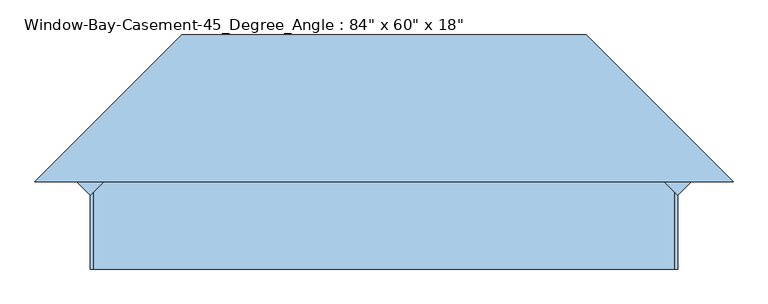
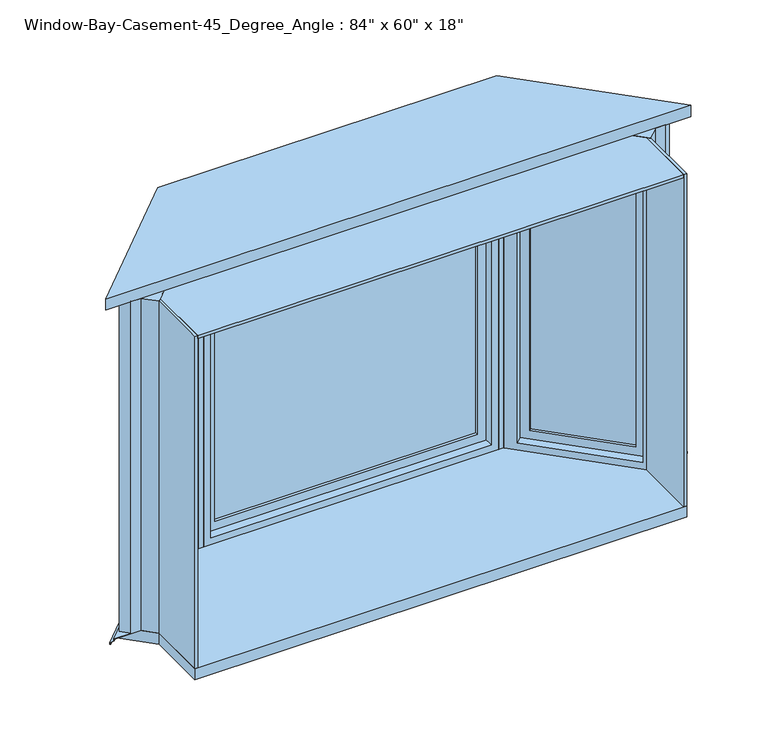
"""IFC4 building model written with IfcOpenShell, lengths in millimetres: window geometry."""

from ifc_helpers import new_model, si_unit, frame, origin, place, context, project, spatial, polyline, outline, extrude, faceted_brep, source, transform, mapped, element, save


def window_a80803ce(model_context):
    return source(origin(), model_context, "Body", "SolidModel", [
        extrude(outline(polyline([(1066.8, 208.1414087), (1062.3098719, 203.6512806), (771.5637138, 494.3974388), (776.0538418, 498.8875668), (1066.8, 208.1414087)])), frame((0.0, 0.0, 730.25), z_axis=(0.0, 0.0, 1.0), x_axis=(1.0, 0.0, 0.0)), (0.0, 0.0, 1.0), 1384.3),
        extrude(outline(polyline([(1057.8197439, 199.1611525), (1053.3296158, 194.6710245), (762.5834576, 485.4171827), (767.0735857, 489.9073107), (1057.8197439, 199.1611525)])), frame((0.0, 0.0, 730.25), z_axis=(0.0, 0.0, 1.0), x_axis=(1.0, 0.0, 0.0)), (0.0, 0.0, 1.0), 1384.3),
        extrude(outline(polyline([(1441.45, 57.15), (1441.45, -468.3271601), (-57.15, -468.3271601), (-57.15, 57.15), (1441.45, 57.15)]), holes=[polyline([(1384.3, -411.1771601), (1384.3, 0.0), (0.0, 0.0), (0.0, -411.1771601), (1384.3, -411.1771601)])]), frame((1044.3493597, 185.6907684, 730.25), z_axis=(0.7071067811865468, 0.7071067811865483, 0.0), x_axis=(0.0, 0.0, 1.0)), (0.0, 0.0, 1.0), 44.45),
        faceted_brep([(661.8085913, 514.35, 2184.4), (1066.8, 109.3585913, 2184.4), (1116.1914087, 158.75, 2184.4), (1161.0926893, 158.75, 2184.4), (703.8926893, 615.95, 2184.4), (1084.7605122, 145.2796158, 2171.7), (713.192049, 516.8480791, 2171.7), (758.0933296, 561.7493597, 2171.7), (1129.6617928, 190.1808964, 2171.7), (1044.3493597, 131.8092316, 2152.65), (699.7216648, 476.4369265, 2152.65), (726.6624332, 503.3776949, 2152.65), (1071.2901281, 158.75, 2152.65), (713.192049, 516.8480791, 673.1), (758.0933296, 561.7493597, 673.1), (699.7216648, 476.4369265, 692.15), (726.6624332, 503.3776949, 692.15), (703.8926893, 615.95, 660.4), (1161.0926893, 158.75, 660.4), (1116.1914087, 158.75, 660.4), (1066.8, 109.3585913, 660.4), (661.8085913, 514.35, 660.4), (1084.7605122, 145.2796158, 673.1), (1129.6617928, 190.1808964, 673.1), (1044.3493597, 131.8092316, 692.15), (1071.2901281, 158.75, 692.15)], [[[0, 1, 2, 3, 4]], [[5, 6, 7, 8]], [[9, 10, 11, 12]], [[6, 13, 14, 7]], [[10, 15, 16, 11]], [[17, 18, 19, 20, 21]], [[13, 22, 23, 14]], [[15, 24, 25, 16]], [[20, 19, 2, 1]], [[3, 18, 17, 4], [7, 14, 23, 8]], [[8, 23, 22, 5]], [[5, 22, 13, 6], [11, 16, 25, 12]], [[12, 25, 24, 9]], [[1, 0, 21, 20], [9, 24, 15, 10]], [[4, 17, 21, 0]], [[2, 19, 18, 3]]]),
        extrude(outline(polyline([(-1066.8, 208.1414087), (-776.0538418, 498.8875668), (-771.5637138, 494.3974388), (-1062.3098719, 203.6512806), (-1066.8, 208.1414087)])), frame((0.0, 0.0, 730.25), z_axis=(0.0, 0.0, 1.0), x_axis=(1.0, 0.0, 0.0)), (0.0, 0.0, 1.0), 1384.3),
        extrude(outline(polyline([(-1057.8197439, 199.1611525), (-767.0735857, 489.9073107), (-762.5834576, 485.4171827), (-1053.3296158, 194.6710245), (-1057.8197439, 199.1611525)])), frame((0.0, 0.0, 730.25), z_axis=(0.0, 0.0, 1.0), x_axis=(1.0, 0.0, 0.0)), (0.0, 0.0, 1.0), 1384.3),
        extrude(outline(polyline([(1441.45, -57.15), (-57.15, -57.15), (-57.15, 468.3271601), (1441.45, 468.3271601), (1441.45, -57.15)]), holes=[polyline([(1384.3, 411.1771601), (0.0, 411.1771601), (0.0, 0.0), (1384.3, 0.0), (1384.3, 411.1771601)])]), frame((-1044.3493597, 185.6907684, 730.25), z_axis=(-0.7071067811865468, 0.7071067811865483, 0.0), x_axis=(0.0, 0.0, 1.0)), (0.0, 0.0, 1.0), 44.45),
        faceted_brep([(-661.8085913, 514.35, 2184.4), (-703.8926893, 615.95, 2184.4), (-1161.0926893, 158.75, 2184.4), (-1116.1914087, 158.75, 2184.4), (-1066.8, 109.3585913, 2184.4), (-1084.7605122, 145.2796158, 2171.7), (-1129.6617928, 190.1808964, 2171.7), (-758.0933296, 561.7493597, 2171.7), (-713.192049, 516.8480791, 2171.7), (-1044.3493597, 131.8092316, 2152.65), (-1071.2901281, 158.75, 2152.65), (-726.6624332, 503.3776949, 2152.65), (-699.7216648, 476.4369265, 2152.65), (-758.0933296, 561.7493597, 673.1), (-713.192049, 516.8480791, 673.1), (-726.6624332, 503.3776949, 692.15), (-699.7216648, 476.4369265, 692.15), (-703.8926893, 615.95, 660.4), (-661.8085913, 514.35, 660.4), (-1066.8, 109.3585913, 660.4), (-1116.1914087, 158.75, 660.4), (-1161.0926893, 158.75, 660.4), (-1129.6617928, 190.1808964, 673.1), (-1084.7605122, 145.2796158, 673.1), (-1071.2901281, 158.75, 692.15), (-1044.3493597, 131.8092316, 692.15)], [[[0, 1, 2, 3, 4]], [[5, 6, 7, 8]], [[9, 10, 11, 12]], [[8, 7, 13, 14]], [[12, 11, 15, 16]], [[17, 18, 19, 20, 21]], [[14, 13, 22, 23]], [[16, 15, 24, 25]], [[19, 4, 3, 20]], [[2, 1, 17, 21], [7, 6, 22, 13]], [[6, 5, 23, 22]], [[5, 8, 14, 23], [11, 10, 24, 15]], [[10, 9, 25, 24]], [[4, 19, 18, 0], [9, 12, 16, 25]], [[1, 0, 18, 17]], [[3, 2, 21, 20]]]),
        faceted_brep([(-724.9347382, 666.75, 660.4), (-724.9347382, 666.75, 653.0697935), (724.9347382, 666.75, 653.0697935), (724.9347382, 666.75, 660.4), (-703.8926893, 615.95, 663.1486341), (-703.8926893, 615.95, 660.4), (703.8926893, 615.95, 660.4), (703.8926893, 615.95, 663.1486341), (-725.5133946, 668.147, 654.4483503), (-725.5133946, 668.147, 663.1486341), (725.5133946, 668.147, 663.1486341), (725.5133946, 668.147, 654.4483503), (730.7739068, 680.847, 652.2089977), (-730.7739068, 680.847, 652.2089977), (730.7739068, 680.847, 643.2668038), (-730.7739068, 680.847, 643.2668038), (-729.132627, 676.8846, 644.7270038), (-729.132627, 676.8846, 643.2668038), (729.132627, 676.8846, 643.2668038), (729.132627, 676.8846, 644.7270038), (-730.1110823, 679.2468, 650.8662705), (-730.1110823, 679.2468, 644.7270038), (730.1110823, 679.2468, 644.7270038), (730.1110823, 679.2468, 650.8662705), (-1232.9347382, 158.75, 660.4), (-1232.9347382, 158.75, 653.0697935), (1232.9347382, 158.75, 660.4), (1161.0926893, 158.75, 660.4), (-1161.0926893, 158.75, 660.4), (-1161.0926893, 158.75, 663.1486341), (1161.0926893, 158.75, 663.1486341), (1234.9103945, 158.75, 663.1486341), (-1234.9103945, 158.75, 663.1486341), (-1234.9103945, 158.75, 654.4483503), (-1252.8709068, 158.75, 652.2089977), (-1252.8709068, 158.75, 643.2668038), (1252.8709068, 158.75, 643.2668038), (1247.2672271, 158.75, 643.2668038), (-1247.2672271, 158.75, 643.2668038), (-1247.2672271, 158.75, 644.7270038), (1247.2672271, 158.75, 644.7270038), (1250.6078823, 158.75, 644.7270038), (-1250.6078823, 158.75, 644.7270038), (-1250.6078823, 158.75, 650.8662705), (1232.9347382, 158.75, 653.0697935), (1234.9103945, 158.75, 654.4483503), (1252.8709068, 158.75, 652.2089977), (1250.6078823, 158.75, 650.8662705)], [[[0, 1, 2, 3]], [[4, 5, 6, 7]], [[8, 9, 10, 11]], [[8, 11, 12, 13]], [[13, 12, 14, 15]], [[16, 17, 18, 19]], [[20, 21, 22, 23]], [[2, 1, 20, 23]], [[1, 0, 24, 25]], [[0, 3, 26, 27, 6, 5, 28, 24]], [[5, 4, 29, 28]], [[4, 7, 30, 31, 10, 9, 32, 29]], [[9, 8, 33, 32]], [[8, 13, 34, 33]], [[13, 15, 35, 34]], [[15, 14, 36, 37, 18, 17, 38, 35]], [[17, 16, 39, 38]], [[16, 19, 40, 41, 22, 21, 42, 39]], [[21, 20, 43, 42]], [[20, 1, 25, 43]], [[3, 2, 44, 26]], [[7, 6, 27, 30]], [[11, 10, 31, 45]], [[12, 11, 45, 46]], [[14, 12, 46, 36]], [[19, 18, 37, 40]], [[23, 22, 41, 47]], [[2, 23, 47, 44]], [[25, 24, 28, 29, 32, 33, 34, 35, 38, 39, 42, 43]], [[27, 26, 44, 47, 41, 40, 37, 36, 46, 45, 31, 30]]]),
        extrude(outline(polyline([(-1138.642049, 181.2006403), (-1161.0926893, 158.75), (-1192.5235857, 190.1808964), (-1170.0729454, 212.6315367), (-1138.642049, 181.2006403)])), frame((0.0, 0.0, 663.1486341), z_axis=(0.0, 0.0, 1.0), x_axis=(1.0, 0.0, 0.0)), (0.0, 0.0, 1.0), 1521.2513659),
        extrude(outline(polyline([(1138.642049, 181.2006403), (1170.0729454, 212.6315367), (1192.5235857, 190.1808964), (1161.0926893, 158.75), (1138.642049, 181.2006403)])), frame((0.0, 0.0, 663.1486341), z_axis=(0.0, 0.0, 1.0), x_axis=(1.0, 0.0, 0.0)), (0.0, 0.0, 1.0), 1521.2513659),
        extrude(outline(polyline([(-661.8085913, 514.35), (661.8085913, 514.35), (1054.1, 122.0585913), (1054.1, -158.75), (-1054.1, -158.75), (-1054.1, 122.0585913), (-661.8085913, 514.35)])), frame((0.0, 0.0, 2171.7), z_axis=(0.0, 0.0, 1.0), x_axis=(1.0, 0.0, 0.0)), (0.0, 0.0, 1.0), 12.7),
        extrude(outline(polyline([(-1066.8, -158.75), (-1066.8, 109.3585913), (-1054.1, 122.0585913), (-1054.1, -158.75), (-1066.8, -158.75)])), frame((0.0, 0.0, 660.4), z_axis=(0.0, 0.0, 1.0), x_axis=(1.0, 0.0, 0.0)), (0.0, 0.0, 1.0), 1524.0),
        extrude(outline(polyline([(1066.8, -158.75), (1054.1, -158.75), (1054.1, 122.0585913), (1066.8, 109.3585913), (1066.8, -158.75)])), frame((0.0, 0.0, 660.4), z_axis=(0.0, 0.0, 1.0), x_axis=(1.0, 0.0, 0.0)), (0.0, 0.0, 1.0), 1524.0),
        extrude(outline(polyline([(2171.7, -627.2414087), (673.1, -627.2414087), (673.1, 627.2414087), (2171.7, 627.2414087), (2171.7, -627.2414087)]), holes=[polyline([(2114.55, 570.0914087), (730.25, 570.0914087), (730.25, -570.0914087), (2114.55, -570.0914087), (2114.55, 570.0914087)])]), frame((0.0, 552.45, 0.0), z_axis=(0.0, 1.0, 0.0), x_axis=(0.0, 0.0, 1.0)), (0.0, 0.0, 1.0), 44.45),
        extrude(outline(polyline([(1066.8, -158.75), (-1066.8, -158.75), (-1066.8, 109.3585913), (-1174.5630735, 217.1216648), (-724.9347382, 666.75), (724.9347382, 666.75), (1174.5630735, 217.1216648), (1066.8, 109.3585913), (1066.8, -158.75)])), frame((0.0, 0.0, 609.6), z_axis=(0.0, 0.0, 1.0), x_axis=(1.0, 0.0, 0.0)), (0.0, 0.0, 1.0), 50.8),
        extrude(outline(polyline([(570.0914087, 584.2), (570.0914087, 577.85), (-570.0914087, 577.85), (-570.0914087, 584.2), (570.0914087, 584.2)])), frame((0.0, 0.0, 730.25), z_axis=(0.0, 0.0, 1.0), x_axis=(1.0, 0.0, 0.0)), (0.0, 0.0, 1.0), 1384.3),
        extrude(outline(polyline([(570.0914087, 571.5), (570.0914087, 565.15), (-570.0914087, 565.15), (-570.0914087, 571.5), (570.0914087, 571.5)])), frame((0.0, 0.0, 730.25), z_axis=(0.0, 0.0, 1.0), x_axis=(1.0, 0.0, 0.0)), (0.0, 0.0, 1.0), 1384.3),
        faceted_brep([(627.2414087, 552.45, 673.1), (627.2414087, 615.95, 673.1), (-627.2414087, 615.95, 673.1), (-627.2414087, 552.45, 673.1), (608.1914087, 514.35, 692.15), (608.1914087, 552.45, 692.15), (-608.1914087, 552.45, 692.15), (-608.1914087, 514.35, 692.15), (639.9414087, 615.95, 660.4), (639.9414087, 514.35, 660.4), (-639.9414087, 514.35, 660.4), (-639.9414087, 615.95, 660.4), (-627.2414087, 615.95, 2171.7), (-627.2414087, 552.45, 2171.7), (-608.1914087, 552.45, 2152.65), (-608.1914087, 514.35, 2152.65), (-639.9414087, 514.35, 2184.4), (-639.9414087, 615.95, 2184.4), (627.2414087, 615.95, 2171.7), (627.2414087, 552.45, 2171.7), (608.1914087, 552.45, 2152.65), (608.1914087, 514.35, 2152.65), (639.9414087, 514.35, 2184.4), (639.9414087, 615.95, 2184.4)], [[[0, 1, 2, 3]], [[4, 5, 6, 7]], [[8, 9, 10, 11]], [[3, 2, 12, 13]], [[7, 6, 14, 15]], [[11, 10, 16, 17]], [[13, 12, 18, 19]], [[15, 14, 20, 21]], [[17, 16, 22, 23]], [[11, 17, 23, 8], [1, 18, 12, 2]], [[19, 18, 1, 0]], [[3, 13, 19, 0], [5, 20, 14, 6]], [[21, 20, 5, 4]], [[9, 22, 16, 10], [7, 15, 21, 4]], [[23, 22, 9, 8]]]),
        extrude(outline(polyline([(-639.9414087, 615.95), (-639.9414087, 514.35), (-661.8085913, 514.35), (-703.8926893, 615.95), (-639.9414087, 615.95)])), frame((0.0, 0.0, 660.4), z_axis=(0.0, 0.0, 1.0), x_axis=(1.0, 0.0, 0.0)), (0.0, 0.0, 1.0), 1524.0),
        extrude(outline(polyline([(703.8926893, 615.95), (661.8085913, 514.35), (639.9414087, 514.35), (639.9414087, 615.95), (703.8926893, 615.95)])), frame((0.0, 0.0, 660.4), z_axis=(0.0, 0.0, 1.0), x_axis=(1.0, 0.0, 0.0)), (0.0, 0.0, 1.0), 1524.0),
        extrude(outline(polyline([(735.4557627, 692.15), (1268.8557627, 158.75), (-1268.8557627, 158.75), (-735.4557627, 692.15), (735.4557627, 692.15)])), frame((0.0, 0.0, 2184.4), z_axis=(0.0, 0.0, 1.0), x_axis=(1.0, 0.0, 0.0)), (0.0, 0.0, 1.0), 50.8),
    ])


if __name__ == "__main__":
    model = new_model("IFC4")
    model_context = context("Model", 3, world=origin())
    ifc_project = project(units=[si_unit("LENGTHUNIT", "METRE", prefix="MILLI")], contexts=[model_context])
    site = spatial("IfcSite", under=ifc_project)
    building = spatial("IfcBuilding", under=site)
    placement = place(None, origin())
    window_shape = window_a80803ce(model_context)
    element("IfcWindow", 1, ObjectType="Window-Bay-Casement-45_Degree_Angle : 84\" x 60\" x 18\"", at=placement, inside=building, context=model_context, shape_type="MappedRepresentation", body=[
        mapped(window_shape, transform((0.0, 0.0, 0.0), x_axis=(1.0, 0.0, 0.0), y_axis=(0.0, 1.0, 0.0), z_axis=(0.0, 0.0, 1.0))),
    ])
    save(model, "model.ifc")

# Revit data of these elements
# Type "Window-Bay-Casement-45_Degree_Angle : 84\" x 60\" x 18\""
#   Type Mark = "27"
#   Fire Rating = "0.5h"
#   Assembly Code = "B2020100"
#   Analytic Construction = "Double glazing - domestic"
#   Width of Middle Sash = 4' - 2.38909"
#   Width = 7' - 0"
#   Visual Light Transmittance = 0.81
#   Thermal Resistance (R) = 1.8146 (h·ft²·°F)/BTU
#   Solar Heat Gain Coefficient = 0.76
#   Rough Width = 7' - 0 1/2"
#   Rough Height = 5' - 0 1/2"
#   Length 4 = 0' - 1.13909"
#   Length 3 = 0' - 0.51777"
#   Length 2 = 4' - 7.42462"
#   Length 1 = 1' - 2.80546"
#   Wall Thickness [instance default] = 0' - 6"
#   Trim Width = 7' - 5.03553"
#   Trim Height = 5' - 0"
#   Height 1 = 5' - 2"
#   Height = 5' - 0"
#   Heat Transfer Coefficient (U) = 0.5511 BTU/(h·ft²·°F)
#   Depth = 1' - 6"
#   Default Sill Height = 2' - 0"
#   Angle 1 = 22.5000°
#   Angle = 45.0000°
#   Center Muntin Visibility = yes
#   Side Muntin Visibility = yes
#   Interior Trim Visibility [instance default] = yes
#   Exterior Trim Visibility [instance default] = yes
#   Center Muntin Pattern = Muntin Pattern_2x2 : Muntin Pattern_2x2
#   Side Muntin Pattern = Muntin Pattern_2x2 : Muntin Pattern_2x2
#   Interior Trim Material = Wood - Stained
#   Exterior Trim Material = Clad - White
#   Exterior Trim = element 422174
#   Interior Trim = Trim-Window-Interior-Flat : Picture Frame
#   Interior Frame Material = Wood - Stained
#   Glass Panel Material = Glass
#   Exterior Frame Material = Clad - White
#   Wall Closure = (empty or 0)
# Element 1 (IfcWindow, "Window-Bay-Casement-45_Degree_Angle : 84\" x 60\" x 18\"")
#   Wall Thickness = 1' - 0 1/2"
#   Materials on its faces: "Wood - Stained", "Clad - White", "Glass"
# Materials
#   "Wood - Stained": class "Wood", colour RGB 224 178 126, transparency 0, Cost = 0
#   "Clad - White": class "Wood", colour RGB 245 245 243, transparency 0, Cost = 0
#   "Glass": class "Glass", colour RGB 0 128 192, transparency 0.75, Description = "Soda Lime Glass", Cost = 0
